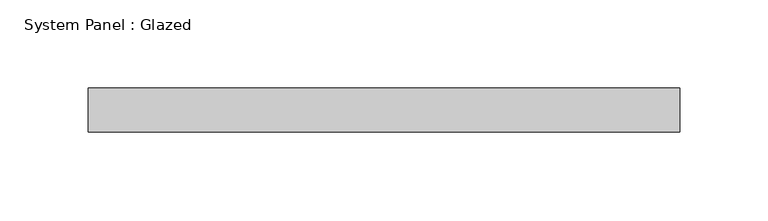
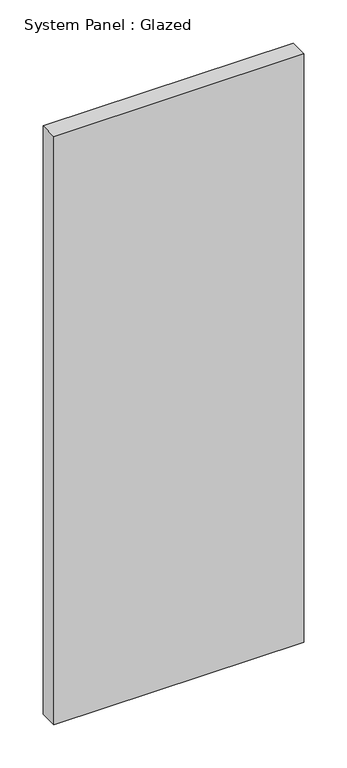
"""IFC4 building model written with IfcOpenShell, lengths in millimetres: plate geometry, System Panel : Glazed."""

from ifc_helpers import new_model, si_unit, origin, origin_with_axes, place, context, project, spatial, polyline, outline, extrude, source, transform, mapped, element, save


def system_panel_glazed_7d21766c(model_context):
    return source(origin(), model_context, "Body", "SweptSolid", [
        extrude(outline(polyline([(167.4242424, 24.5), (-167.4242424, 24.5), (-167.4242424, 49.5), (167.4242424, 49.5), (167.4242424, 24.5)])), origin_with_axes(), (0.0, 0.0, 1.0), 833.3333333),
    ])


if __name__ == "__main__":
    model = new_model("IFC4")
    model_context = context("Model", 3, world=origin())
    ifc_project = project(units=[si_unit("LENGTHUNIT", "METRE", prefix="MILLI")], contexts=[model_context])
    site = spatial("IfcSite", under=ifc_project)
    building = spatial("IfcBuilding", under=site)
    placement = place(None, origin())
    system_panel_glazed_shape = system_panel_glazed_7d21766c(model_context)
    element("IfcPlate", 1, ObjectType="System Panel : Glazed", at=placement, inside=building, context=model_context, shape_type="MappedRepresentation", body=[
        mapped(system_panel_glazed_shape, transform((0.0, 0.0, 0.0), x_axis=(1.0, 0.0, 0.0), y_axis=(0.0, 1.0, 0.0), z_axis=(0.0, 0.0, 1.0))),
    ])
    save(model, "model.ifc")

# Revit data of these elements
# Element 1 (IfcPlate, "System Panel : Glazed")
#   Materials on its faces: "Glass"
# Materials
#   "Glass": class "Glass", colour RGB 218 227 224, transparency 0.85, Description = "Soda Lime Glass", Cost = 0
